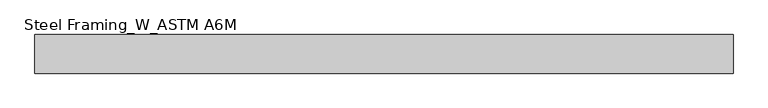
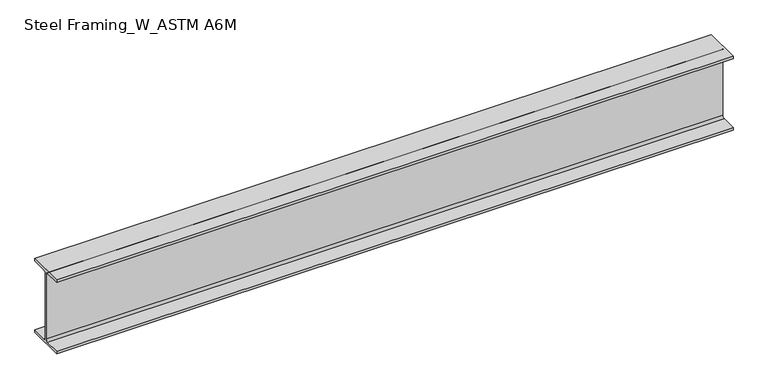
"""IFC4 building model written with IfcOpenShell, lengths in millimetres: beam geometry, Steel Framing_W_ASTM A6M : H_SB_AR_S02_W360x51_G3."""

from ifc_helpers import new_model, si_unit, point, frame, frame_2d, origin, place, context, project, spatial, polyline, circle_curve, trimmed, segment, composite_curve, outline, extrude, source, transform, mapped, element, save


def steel_framing_w_astm_a6m_e4ca242c(model_context):
    return source(origin(), model_context, "Body", "SweptSolid", [
        extrude(outline(composite_curve([segment(polyline([(85.5, -166.4), (85.5, -178.0), (-85.5, -178.0), (-85.5, -166.4), (-13.72, -166.4)]), True, "CONTINUOUS"), segment(trimmed(circle_curve(frame_2d((-13.72, -156.3)), 10.1), [point((-13.72, -166.4))], [point((-3.62, -156.3))], True, "CARTESIAN"), True, "CONTINUOUS"), segment(polyline([(-3.62, -156.3), (-3.62, 156.3)]), True, "CONTINUOUS"), segment(trimmed(circle_curve(frame_2d((-13.72, 156.3)), 10.1), [point((-3.62, 156.3))], [point((-13.72, 166.4))], True, "CARTESIAN"), True, "CONTINUOUS"), segment(polyline([(-13.72, 166.4), (-85.5, 166.4), (-85.5, 178.0), (85.5, 178.0), (85.5, 166.4), (13.72, 166.4)]), True, "CONTINUOUS"), segment(trimmed(circle_curve(frame_2d((13.72, 156.3)), 10.1), [point((13.72, 166.4))], [point((3.62, 156.3))], True, "CARTESIAN"), True, "CONTINUOUS"), segment(polyline([(3.62, 156.3), (3.62, -156.3)]), True, "CONTINUOUS"), segment(trimmed(circle_curve(frame_2d((13.72, -156.3)), 10.1), [point((3.62, -156.3))], [point((13.72, -166.4))], True, "CARTESIAN"), True, "CONTINUOUS"), segment(polyline([(13.72, -166.4), (85.5, -166.4)]), True, "CONTINUOUS")], self_intersect=False)), frame((-1487.2, 0.0, 0.0), z_axis=(1.0, 0.0, 0.0), x_axis=(0.0, 1.0, 0.0)), (0.0, 0.0, 1.0), 3087.7),
    ])


if __name__ == "__main__":
    model = new_model("IFC4")
    model_context = context("Model", 3, world=origin())
    ifc_project = project(units=[si_unit("LENGTHUNIT", "METRE", prefix="MILLI")], contexts=[model_context])
    site = spatial("IfcSite", under=ifc_project)
    building = spatial("IfcBuilding", under=site)
    placement = place(None, origin())
    steel_framing_w_astm_a6m_shape = steel_framing_w_astm_a6m_e4ca242c(model_context)
    element("IfcBeam", 1, ObjectType="Steel Framing_W_ASTM A6M : H_SB_AR_S02_W360x51_G3", at=placement, inside=building, context=model_context, shape_type="MappedRepresentation", body=[
        mapped(steel_framing_w_astm_a6m_shape, transform((0.0, 0.0, 0.0), x_axis=(1.0, 0.0, 0.0), y_axis=(0.0, 1.0, 0.0), z_axis=(0.0, 0.0, 1.0))),
    ])
    save(model, "model.ifc")

# Revit data of these elements
# Type "Steel Framing_W_ASTM A6M : H_SB_AR_S02_W360x51_G3"
#   Type Mark = "G3"
#   Section Name Key = "W14x34"
#   Width = 17.1 cm
#   Web Thickness = 0.724 cm
#   Web Fillet = 1.01 cm
#   Warping Constant = 287000.0 cm⁶
#   Torsional Moment of Inertia = 23.70 cm⁴
#   Section Area = 64.5 cm²
#   Plastic Modulus weak axis = 174.0 cm³
#   Plastic Modulus strong axis = 895.0 cm³
#   Perimeter = 1.36 m²/m
#   Nominal Weight = 51.00 kgf/m
#   Moment of Inertia weak axis = 970.00 cm⁴
#   Moment of Inertia strong axis = 14200.00 cm⁴
#   Height = 35.6 cm
#   Flange Thickness = 1.16 cm
#   Elastic Modulus weak axis = 113.0 cm³
#   Elastic Modulus strong axis = 796.0 cm³
#   Centroid Vertical = 17.8 cm
#   Centroid Horizontal = 8.55 cm
#   Length [instance default] = 1500 mm
#   Structural Material [instance default] = Steel, 45-345
#   Bolt Spacing = 0
#   Assembly Code = ""
# Element 1 (IfcBeam, "Steel Framing_W_ASTM A6M : H_SB_AR_S02_W360x51_G3")
#   Materials on its faces: "Steel, 45-345"
# Materials
#   "Steel, 45-345": class "Metal", colour RGB 189 187 185, transparency 0, Description = "Steel 345 MPa", Cost = 0
